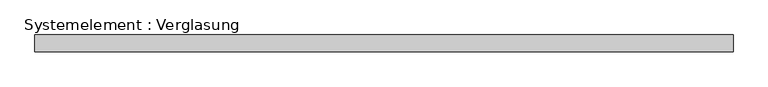
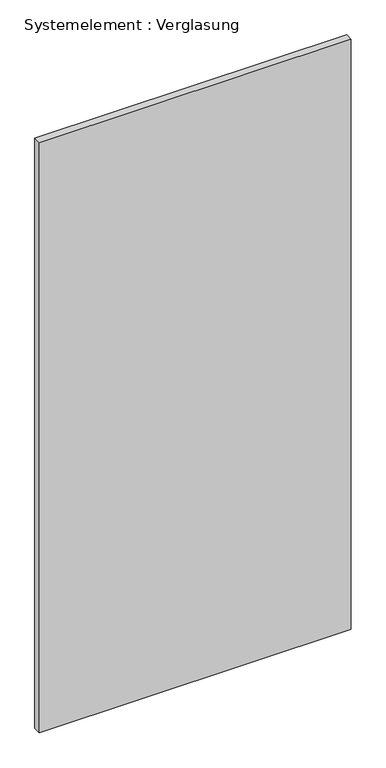
"""IFC4 building model written with IfcOpenShell, lengths in millimetres: plate geometry, Systemelement : Verglasung."""

from ifc_helpers import new_model, si_unit, origin, origin_with_axes, place, context, project, spatial, polyline, outline, extrude, source, transform, mapped, element, save


def systemelement_verglasung_a16edcf7(model_context):
    return source(origin(), model_context, "Body", "SweptSolid", [
        extrude(outline(polyline([(625.0000002, -15.0), (-625.0000002, -15.0), (-625.0000002, 15.0), (625.0000002, 15.0), (625.0000002, -15.0)])), origin_with_axes(), (0.0, 0.0, 1.0), 2500.0),
    ])


if __name__ == "__main__":
    model = new_model("IFC4")
    model_context = context("Model", 3, world=origin())
    ifc_project = project(units=[si_unit("LENGTHUNIT", "METRE", prefix="MILLI")], contexts=[model_context])
    site = spatial("IfcSite", under=ifc_project)
    building = spatial("IfcBuilding", under=site)
    placement = place(None, origin())
    systemelement_verglasung_shape = systemelement_verglasung_a16edcf7(model_context)
    element("IfcPlate", 1, ObjectType="Systemelement : Verglasung", at=placement, inside=building, context=model_context, shape_type="MappedRepresentation", body=[
        mapped(systemelement_verglasung_shape, transform((0.0, 0.0, 0.0), x_axis=(1.0, 0.0, 0.0), y_axis=(0.0, 1.0, 0.0), z_axis=(0.0, 0.0, 1.0))),
    ])
    save(model, "model.ifc")

# Revit data of these elements
# Type "Systemelement : Verglasung"
#   Construction Type Id = "GSP4R"
#   Analytic Construction = "1/8 Zoll Pilkington-Verglasung einfach"
#   Visual Light Transmittance = 0.9
#   Solar Heat Gain Coefficient = 0.86
#   Heat Transfer Coefficient (U) = 6.7069 W/(m²·K)
# Element 1 (IfcPlate, "Systemelement : Verglasung")
#   Materials on its faces: "Glas"
# Materials
#   "Glas": class "Glas", colour RGB 0 0 255, transparency 0.75, Comments = "Render-Darstellung nicht aktualisiert ", Cost = 0
